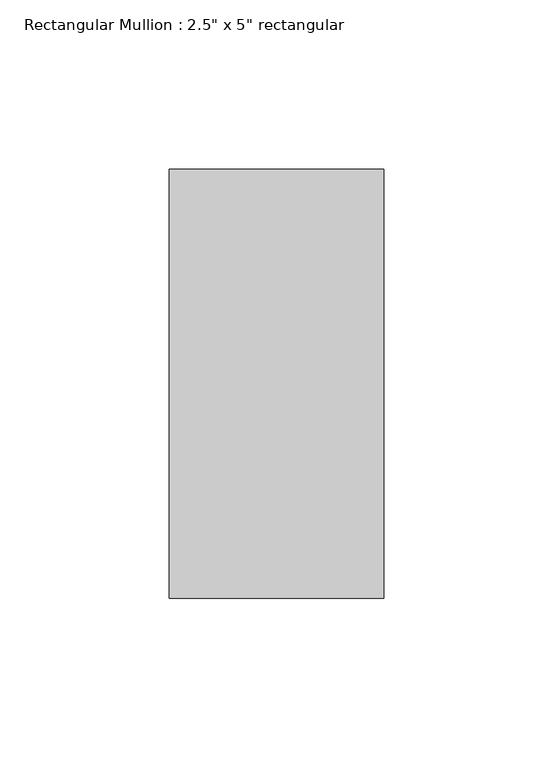
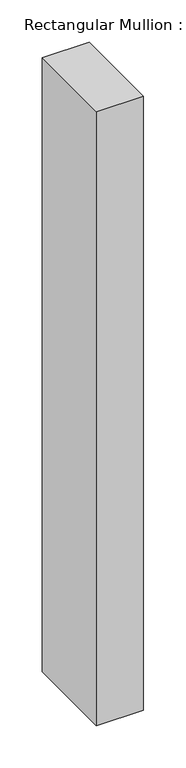
"""IFC4 building model written with IfcOpenShell, lengths in millimetres: member geometry."""

import ifcopenshell
import ifcopenshell.guid

model = None  # the IFC model being written
_history = None  # IfcOwnerHistory: only IFC2X3 demands one
_inside = {}  # id of a spatial element -> (the spatial element, [elements in it])
_under = {}  # id of a project, library or spatial element -> (it, [spatial elements below it])
_declared = {}  # id of a project -> (the project, [libraries it declares])
_typed = {}  # id of a type object -> (the type object, [elements of that type])
_made_of = {}  # id of a material, layer set ... -> (it, [elements and type objects made of it])


def new_model(schema):
    """Start an empty IFC model of exactly this schema.

    Asked for "IFC4X3", IfcOpenShell would pick the latest addendum, in which some entities
    have other attributes; the version numbers below select the first issue.
    IFC2X3 requires an IfcOwnerHistory on every rooted entity: one is made here for all.
    """
    global model, _history
    if schema == "IFC4X3":
        model = ifcopenshell.file(schema_version=(4, 3, 0, 0))
    else:
        model = ifcopenshell.file(schema=schema)
    _inside.clear()
    _under.clear()
    _declared.clear()
    _typed.clear()
    _made_of.clear()
    _history = None
    if model.schema == "IFC2X3":
        org = make("IfcOrganization", Name="unknown")
        user = make(
            "IfcPersonAndOrganization",
            ThePerson=make("IfcPerson", FamilyName="unknown"),
            TheOrganization=org,
        )
        app = make(
            "IfcApplication",
            ApplicationDeveloper=org,
            Version="unknown",
            ApplicationFullName="unknown",
            ApplicationIdentifier="unknown",
        )
        _history = make(
            "IfcOwnerHistory",
            OwningUser=user,
            OwningApplication=app,
            ChangeAction="ADDED",
            CreationDate=0,
        )
    return model


def make(cls, **values):
    """One entity of the class cls with the attributes given. An attribute that is None is left unset."""
    return model.create_entity(
        cls, **{name: value for name, value in values.items() if value is not None}
    )


def rooted(cls, **values):
    """An entity with a GlobalId (a new one), such as an element, a storey or a relation."""
    return make(cls, GlobalId=ifcopenshell.guid.new(), OwnerHistory=_history, **values)


def si_unit(unit_type, name, prefix=None):
    """IfcSIUnit, for example si_unit("LENGTHUNIT", "METRE", prefix="MILLI")."""
    return make("IfcSIUnit", UnitType=unit_type, Prefix=prefix, Name=name)


def assignment(units):
    """IfcUnitAssignment: the units of a project."""
    return None if units is None else make("IfcUnitAssignment", Units=units)


def point(xyz):
    """IfcCartesianPoint."""
    return None if xyz is None else make("IfcCartesianPoint", Coordinates=xyz)


def direction(xyz):
    """IfcDirection."""
    return None if xyz is None else make("IfcDirection", DirectionRatios=xyz)


def frame(location, z_axis=None, x_axis=None):
    """IfcAxis2Placement3D, a coordinate frame: its origin and axes. An axis left out is left unset."""
    return make(
        "IfcAxis2Placement3D",
        Location=point(location),
        Axis=direction(z_axis),
        RefDirection=direction(x_axis),
    )


def origin():
    """The frame at (0, 0, 0) with its axes left unset."""
    return frame((0.0, 0.0, 0.0))


def place(relative_to, where):
    """IfcLocalPlacement: puts the frame where relative to a parent placement (None: the world)."""
    return make(
        "IfcLocalPlacement", PlacementRelTo=relative_to, RelativePlacement=where
    )


def context(
    kind, dimensions, precision=None, world=None, true_north=None, identifier=None
):
    """IfcGeometricRepresentationContext, for example the 3D "Model" context."""
    return make(
        "IfcGeometricRepresentationContext",
        ContextIdentifier=identifier,
        ContextType=kind,
        CoordinateSpaceDimension=dimensions,
        Precision=precision,
        WorldCoordinateSystem=world,
        TrueNorth=true_north,
    )


def project(units=None, contexts=None):
    """IfcProject with its units and contexts."""
    return rooted(
        "IfcProject",
        Name="project",
        RepresentationContexts=contexts,
        UnitsInContext=assignment(units),
    )


def spatial(cls, under=None, at=None, **own):
    """A site, building, storey or space (cls), placed at a placement, below another one or the project."""
    s = rooted(cls, ObjectPlacement=at, **own)
    if under is not None:
        _under.setdefault(under.id(), (under, []))[1].append(s)
    return s


def polyline(points):
    """IfcPolyline through the points."""
    return make("IfcPolyline", Points=[point(p) for p in points])


def outline(outer, holes=None, kind="AREA"):
    """IfcArbitraryClosedProfileDef: a profile drawn as a closed curve; with holes, ...WithVoids."""
    if holes is None:
        return make("IfcArbitraryClosedProfileDef", ProfileType=kind, OuterCurve=outer)
    return make(
        "IfcArbitraryProfileDefWithVoids",
        ProfileType=kind,
        OuterCurve=outer,
        InnerCurves=holes,
    )


def extrude(swept, where, along, depth):
    """IfcExtrudedAreaSolid: the profile swept, set in the frame where, extruded along a direction by depth."""
    return make(
        "IfcExtrudedAreaSolid",
        SweptArea=swept,
        Position=where,
        ExtrudedDirection=direction(along),
        Depth=depth,
    )


def shape(context_of_items, identifier, shape_type, items):
    """IfcShapeRepresentation: the items that make up one representation, for example the "Body"."""
    return make(
        "IfcShapeRepresentation",
        ContextOfItems=context_of_items,
        RepresentationIdentifier=identifier,
        RepresentationType=shape_type,
        Items=items,
    )


def source(mapping_origin, context_of_items, identifier, shape_type, items):
    """IfcRepresentationMap: a shape defined once, which mapped items show again and again."""
    return make(
        "IfcRepresentationMap",
        MappingOrigin=mapping_origin,
        MappedRepresentation=shape(context_of_items, identifier, shape_type, items),
    )


def transform(
    local_origin,
    x_axis=None,
    y_axis=None,
    z_axis=None,
    scale=None,
    scale2=None,
    scale3=None,
    uniform=True,
):
    """IfcCartesianTransformationOperator3D, or its non-uniform kind. x_axis, y_axis, z_axis: its Axis1, 2, 3."""
    if uniform:
        return make(
            "IfcCartesianTransformationOperator3D",
            Axis1=direction(x_axis),
            Axis2=direction(y_axis),
            LocalOrigin=point(local_origin),
            Scale=scale,
            Axis3=direction(z_axis),
        )
    return make(
        "IfcCartesianTransformationOperator3DnonUniform",
        Axis1=direction(x_axis),
        Axis2=direction(y_axis),
        LocalOrigin=point(local_origin),
        Scale=scale,
        Axis3=direction(z_axis),
        Scale2=scale2,
        Scale3=scale3,
    )


def mapped(mapping_source, mapping_target):
    """IfcMappedItem: shows the shape of a source again, moved by a transform."""
    return make(
        "IfcMappedItem", MappingSource=mapping_source, MappingTarget=mapping_target
    )


def made_of(thing, what):
    """Note that an element or type object is made of a material, layer set ...; save() writes the relation."""
    if what is not None:
        _made_of.setdefault(what.id(), (what, []))[1].append(thing)
    return thing


def element(
    cls,
    number,
    at=None,
    inside=None,
    cuts=None,
    type_object=None,
    material=None,
    context=None,
    identifier="Body",
    shape_type=None,
    held_by="IfcProductDefinitionShape",
    body=None,
    shapes=None,
    **own,
):
    """One element of the class cls, such as IfcWall. Its Tag is "e" and its number.

    at: its placement. inside: the storey or other place that contains it. cuts: it is an
    opening in that element (IfcRelVoidsElement). A single representation is given by context,
    identifier, shape_type and body (its items); several are given by shapes. held_by: the class
    of the entity that holds the representations. save() writes the other relations.
    """
    e = rooted(cls, Tag="e%d" % number, ObjectPlacement=at, **own)
    if body is not None:
        shapes = [shape(context, identifier, shape_type, body)]
    if shapes is not None:
        e.Representation = make(held_by, Representations=shapes)
    if inside is not None:
        _inside.setdefault(inside.id(), (inside, []))[1].append(e)
    if cuts is not None:
        rooted(
            "IfcRelVoidsElement", RelatingBuildingElement=cuts, RelatedOpeningElement=e
        )
    if type_object is not None:
        _typed.setdefault(type_object.id(), (type_object, []))[1].append(e)
    return made_of(e, material)


def aggregate(whole, parts):
    """IfcRelAggregates: a whole, such as a stair, and the parts it consists of."""
    return rooted("IfcRelAggregates", RelatingObject=whole, RelatedObjects=parts)


def save(model, path):
    """Write the relations noted so far, then the file.

    IfcRelAggregates (storeys below a building ...), IfcRelContainedInSpatialStructure (elements
    in a storey), IfcRelDefinesByType, IfcRelAssociatesMaterial and IfcRelDeclares: one each for
    every whole, place, type object, material and project.
    """
    for whole, parts in _under.values():
        aggregate(whole, parts)
    for where, things in _inside.values():
        rooted(
            "IfcRelContainedInSpatialStructure",
            RelatedElements=things,
            RelatingStructure=where,
        )
    for kind, things in _typed.values():
        rooted("IfcRelDefinesByType", RelatedObjects=things, RelatingType=kind)
    for what, things in _made_of.values():
        rooted("IfcRelAssociatesMaterial", RelatedObjects=things, RelatingMaterial=what)
    for by, libraries in _declared.values():
        rooted("IfcRelDeclares", RelatingContext=by, RelatedDefinitions=libraries)
    model.write(path)


def member_5cd4c5ac(model_context):
    return source(origin(), model_context, "Body", "SweptSolid", [
        extrude(outline(polyline([(0.0, 63.5), (0.0, -63.5), (-63.5, -63.5), (-63.5, 63.5), (0.0, 63.5)])), frame((0.0, 0.0, -882.65), z_axis=(0.0, 0.0, 1.0), x_axis=(1.0, 0.0, 0.0)), (0.0, 0.0, 1.0), 882.65),
    ])


if __name__ == "__main__":
    model = new_model("IFC4")
    model_context = context("Model", 3, world=origin())
    ifc_project = project(units=[si_unit("LENGTHUNIT", "METRE", prefix="MILLI")], contexts=[model_context])
    site = spatial("IfcSite", under=ifc_project)
    building = spatial("IfcBuilding", under=site)
    placement = place(None, origin())
    member_shape = member_5cd4c5ac(model_context)
    element("IfcMember", 1, ObjectType="Rectangular Mullion : 2.5\" x 5\" rectangular", at=placement, inside=building, context=model_context, shape_type="MappedRepresentation", body=[
        mapped(member_shape, transform((0.0, 0.0, 0.0), x_axis=(1.0, 0.0, 0.0), y_axis=(0.0, 1.0, 0.0), z_axis=(0.0, 0.0, 1.0))),
    ])
    save(model, "model.ifc")

# Revit data of these elements
# Type "Rectangular Mullion : 2.5\" x 5\" rectangular"
#   built-in parameter 1007304 = 0.416667 (stored number, unit not read)
#   built-in parameter 1007301 = 0.104167 (stored number, unit not read)
#   built-in parameter 1007300 = 0.104167 (stored number, unit not read)
# Element 1 (IfcMember, "Rectangular Mullion : 2.5\" x 5\" rectangular")
#   Materials on its faces: "Aluminum"
# Materials
#   "Aluminum": class "Metal", colour RGB 247 247 247, transparency 0, Description = "Aluminum 6061", Cost = 0
